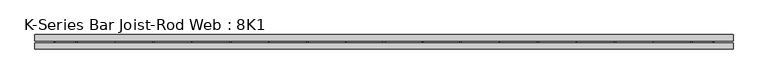
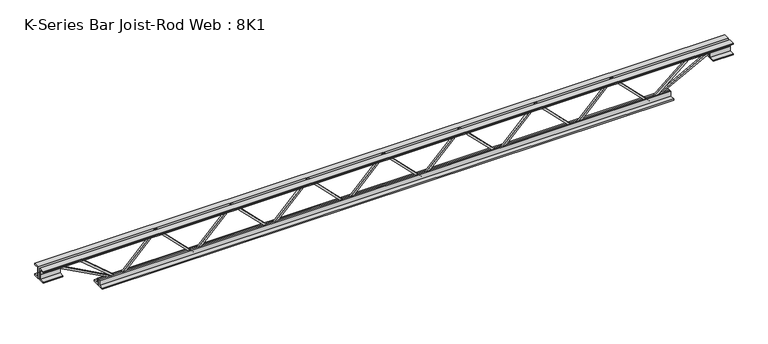
"""IFC4 building model written with IfcOpenShell, lengths in millimetres: beam geometry, K-Series Bar Joist-Rod Web : 8K1."""

from ifc_helpers import new_model, si_unit, frame, origin, place, context, project, spatial, polyline, outline, extrude, source, transform, mapped, element, save


def k_series_bar_joist_rod_web_8k1_f1b48c2f(model_context):
    return source(origin(), model_context, "Body", "SweptSolid", [
        extrude(outline(polyline([(-90.4875, 586.3869215), (-100.0125, 586.3869215), (-100.0125, 591.5448196), (90.4875, 780.6571268), (90.4875, 783.0413306), (-100.0125, 972.1536378), (-100.0125, 977.3115359), (-90.4875, 977.3115359), (-90.4875, 976.119434), (100.0125, 787.0071268), (100.0125, 776.6913306), (-90.4875, 587.5790235), (-90.4875, 586.3869215)])), frame((0.0, -4.7625, 0.0), z_axis=(0.0, 1.0, 0.0), x_axis=(0.0, 0.0, 1.0)), (0.0, 0.0, 1.0), 9.525),
        extrude(outline(polyline([(-90.4875, 195.4623072), (-100.0125, 195.4623072), (-100.0125, 200.6202052), (90.4875, 389.7325124), (90.4875, 392.1167163), (-100.0125, 581.2290235), (-100.0125, 586.3869215), (-90.4875, 586.3869215), (-90.4875, 585.1948196), (100.0125, 396.0825124), (100.0125, 385.7667163), (-90.4875, 196.6544091), (-90.4875, 195.4623072)])), frame((0.0, -4.7625, 0.0), z_axis=(0.0, 1.0, 0.0), x_axis=(0.0, 0.0, 1.0)), (0.0, 0.0, 1.0), 9.525),
        extrude(outline(polyline([(-90.4875, -195.4623072), (-100.0125, -195.4623072), (-100.0125, -190.3044091), (90.4875, -1.1921019), (90.4875, 1.1921019), (-100.0125, 190.3044091), (-100.0125, 195.4623072), (-90.4875, 195.4623072), (-90.4875, 194.2702052), (100.0125, 5.1578981), (100.0125, -5.1578981), (-90.4875, -194.2702052), (-90.4875, -195.4623072)])), frame((0.0, -4.7625, 0.0), z_axis=(0.0, 1.0, 0.0), x_axis=(0.0, 0.0, 1.0)), (0.0, 0.0, 1.0), 9.525),
        extrude(outline(polyline([(-90.4875, -586.3869215), (-100.0125, -586.3869215), (-100.0125, -581.2290235), (90.4875, -392.1167163), (90.4875, -389.7325124), (-100.0125, -200.6202052), (-100.0125, -195.4623072), (-90.4875, -195.4623072), (-90.4875, -196.6544091), (100.0125, -385.7667163), (100.0125, -396.0825124), (-90.4875, -585.1948196), (-90.4875, -586.3869215)])), frame((0.0, -4.7625, 0.0), z_axis=(0.0, 1.0, 0.0), x_axis=(0.0, 0.0, 1.0)), (0.0, 0.0, 1.0), 9.525),
        extrude(outline(polyline([(-90.4875, -977.3115359), (-100.0125, -977.3115359), (-100.0125, -972.1536378), (90.4875, -783.0413306), (90.4875, -780.6571268), (-100.0125, -591.5448196), (-100.0125, -586.3869215), (-90.4875, -586.3869215), (-90.4875, -587.5790235), (100.0125, -776.6913306), (100.0125, -787.0071268), (-90.4875, -976.119434), (-90.4875, -977.3115359)])), frame((0.0, -4.7625, 0.0), z_axis=(0.0, 1.0, 0.0), x_axis=(0.0, 0.0, 1.0)), (0.0, 0.0, 1.0), 9.525),
        extrude(outline(polyline([(-90.4875, 977.3115359), (-100.0125, 977.3115359), (-100.0125, 982.469434), (90.4875, 1171.5817411), (90.4875, 1173.965945), (-100.0125, 1363.0782522), (-100.0125, 1368.2361502), (-90.4875, 1368.2361502), (-90.4875, 1367.0440483), (100.0125, 1177.9317411), (100.0125, 1167.615945), (-90.4875, 978.5036378), (-90.4875, 977.3115359)])), frame((0.0, -4.7625, 0.0), z_axis=(0.0, 1.0, 0.0), x_axis=(0.0, 0.0, 1.0)), (0.0, 0.0, 1.0), 9.525),
        extrude(outline(polyline([(-90.4875, -1368.2361502), (-100.0125, -1368.2361502), (-100.0125, -1363.0782522), (90.4875, -1173.965945), (90.4875, -1171.5817411), (-100.0125, -982.469434), (-100.0125, -977.3115359), (-90.4875, -977.3115359), (-90.4875, -978.5036378), (100.0125, -1167.615945), (100.0125, -1177.9317411), (-90.4875, -1367.0440483), (-90.4875, -1368.2361502)])), frame((0.0, -4.7625, 0.0), z_axis=(0.0, 1.0, 0.0), x_axis=(0.0, 0.0, 1.0)), (0.0, 0.0, 1.0), 9.525),
        extrude(outline(polyline([(4.7625, 101.6), (36.5125, 101.6), (36.5125, 95.25), (11.1125, 95.25), (11.1125, 69.85), (4.7625, 69.85), (4.7625, 101.6)])), frame((-1774.6361502, 0.0, 0.0), z_axis=(1.0, 0.0, 0.0), x_axis=(0.0, 1.0, 0.0)), (0.0, 0.0, 1.0), 3549.2723005),
        extrude(outline(polyline([(-4.7625, 101.6), (-4.7625, 69.85), (-11.1125, 69.85), (-11.1125, 95.25), (-36.5125, 95.25), (-36.5125, 101.6), (-4.7625, 101.6)])), frame((-1774.6361502, 0.0, 0.0), z_axis=(1.0, 0.0, 0.0), x_axis=(0.0, 1.0, 0.0)), (0.0, 0.0, 1.0), 3549.2723005),
        extrude(outline(polyline([(-4.7625, 38.1), (-36.5125, 38.1), (-36.5125, 44.45), (-11.1125, 44.45), (-11.1125, 69.85), (-4.7625, 69.85), (-4.7625, 38.1)])), frame((-1774.6361502, 0.0, 0.0), z_axis=(1.0, 0.0, 0.0), x_axis=(0.0, 1.0, 0.0)), (0.0, 0.0, 1.0), 101.6),
        extrude(outline(polyline([(36.5125, 38.1), (4.7625, 38.1), (4.7625, 69.85), (11.1125, 69.85), (11.1125, 44.45), (36.5125, 44.45), (36.5125, 38.1)])), frame((-1774.6361502, 0.0, 0.0), z_axis=(1.0, 0.0, 0.0), x_axis=(0.0, 1.0, 0.0)), (0.0, 0.0, 1.0), 101.6),
        extrude(outline(polyline([(4.7625, 38.1), (4.7625, 69.85), (11.1125, 69.85), (11.1125, 44.45), (36.5125, 44.45), (36.5125, 38.1), (4.7625, 38.1)])), frame((1673.0361502, 0.0, 0.0), z_axis=(1.0, 0.0, 0.0), x_axis=(0.0, 1.0, 0.0)), (0.0, 0.0, 1.0), 101.6),
        extrude(outline(polyline([(-4.7625, 38.1), (-36.5125, 38.1), (-36.5125, 44.45), (-11.1125, 44.45), (-11.1125, 69.85), (-4.7625, 69.85), (-4.7625, 38.1)])), frame((1673.0361502, 0.0, 0.0), z_axis=(1.0, 0.0, 0.0), x_axis=(0.0, 1.0, 0.0)), (0.0, 0.0, 1.0), 101.6),
        extrude(outline(polyline([(4.7625, -101.6), (4.7625, -69.85), (11.1125, -69.85), (11.1125, -95.25), (36.5125, -95.25), (36.5125, -101.6), (4.7625, -101.6)])), frame((-1469.8361502, 0.0, 0.0), z_axis=(1.0, 0.0, 0.0), x_axis=(0.0, 1.0, 0.0)), (0.0, 0.0, 1.0), 2939.6723005),
        extrude(outline(polyline([(-4.7625, -101.6), (-36.5125, -101.6), (-36.5125, -95.25), (-11.1125, -95.25), (-11.1125, -69.85), (-4.7625, -69.85), (-4.7625, -101.6)])), frame((-1469.8361502, 0.0, 0.0), z_axis=(1.0, 0.0, 0.0), x_axis=(0.0, 1.0, 0.0)), (0.0, 0.0, 1.0), 2939.6723005),
        extrude(outline(polyline([(0.0, -9.525), (0.0, 0.0), (346.6425392, 0.0), (346.6425392, -9.525), (0.0, -9.525)])), frame((-1675.3044487, 4.7625, 65.662372), z_axis=(0.47628314854007936, 0.0, 0.8792919665371388), x_axis=(0.8792919665371388, 0.0, -0.47628314854007936)), (0.0, 0.0, 1.0), 9.525),
        extrude(outline(polyline([(0.0, -9.525), (0.0, 0.0), (255.8584052, 0.0), (255.8584052, -9.525), (0.0, -9.525)])), frame((-1566.7715976, 4.7625, 66.2117016), z_axis=(0.6452787816450547, 0.0, 0.7639471800842477), x_axis=(0.7639471800842477, 0.0, -0.6452787816450547)), (0.0, 0.0, 1.0), 9.525),
        extrude(outline(polyline([(0.0, -9.525), (0.0, 0.0), (346.6425392, 0.0), (346.6425392, -9.525), (0.0, -9.525)])), frame((1675.3044487, -4.7625, 65.662372), z_axis=(-0.4762831485400428, 0.0, 0.8792919665371586), x_axis=(-0.8792919665371586, 0.0, -0.4762831485400428)), (0.0, 0.0, 1.0), 9.525),
        extrude(outline(polyline([(0.0, -9.525), (0.0, 0.0), (255.8584052, 0.0), (255.8584052, -9.525), (0.0, -9.525)])), frame((1566.7715976, -4.7625, 66.2117016), z_axis=(-0.6452787816450276, 0.0, 0.7639471800842706), x_axis=(-0.7639471800842706, 0.0, -0.6452787816450276)), (0.0, 0.0, 1.0), 9.525),
    ])


if __name__ == "__main__":
    model = new_model("IFC4")
    model_context = context("Model", 3, world=origin())
    ifc_project = project(units=[si_unit("LENGTHUNIT", "METRE", prefix="MILLI")], contexts=[model_context])
    site = spatial("IfcSite", under=ifc_project)
    building = spatial("IfcBuilding", under=site)
    placement = place(None, origin())
    k_series_bar_joist_rod_web_8k1_shape = k_series_bar_joist_rod_web_8k1_f1b48c2f(model_context)
    element("IfcBeam", 1, ObjectType="K-Series Bar Joist-Rod Web : 8K1", at=placement, inside=building, context=model_context, shape_type="MappedRepresentation", body=[
        mapped(k_series_bar_joist_rod_web_8k1_shape, transform((0.0, 0.0, 0.0), x_axis=(1.0, 0.0, 0.0), y_axis=(0.0, 1.0, 0.0), z_axis=(0.0, 0.0, 1.0))),
    ])
    save(model, "model.ifc")

# Revit data of these elements
# Type "K-Series Bar Joist-Rod Web : 8K1"
#   Assembly Code = "B1010350"
#   Wt = 5.1
#   Web Thickness = 0' - 0 3/8"
#   Start Offset [instance default] = 0' - 0"
#   Start Extension [instance default] = 0' - 0"
#   Seat Length = 0' - 4"
#   Seat Depth = 0' - 2 1/2"
#   PanelArrayLength [instance default] = 21' - 4"
#   Panel [instance default] = 1' - 4"
#   End Offset [instance default] = 0' - 0"
#   End Extension [instance default] = 0' - 0"
#   End Panel = 1' - 4"
#   Cord Leg = 0' - 1 1/4"
#   Chord Thickness = 0' - 0 1/4"
#   Length [instance default] = 24' - 0"
#   Depth = 0' - 8"
#   PanelArrayNum [instance default] = 16
#   Rendering Material = none
# Element 1 (IfcBeam, "K-Series Bar Joist-Rod Web : 8K1")
#   PanelArrayLength = 8' - 11.73513"
#   Panel = 1' - 3.39073"
#   PanelArrayNum = 7
